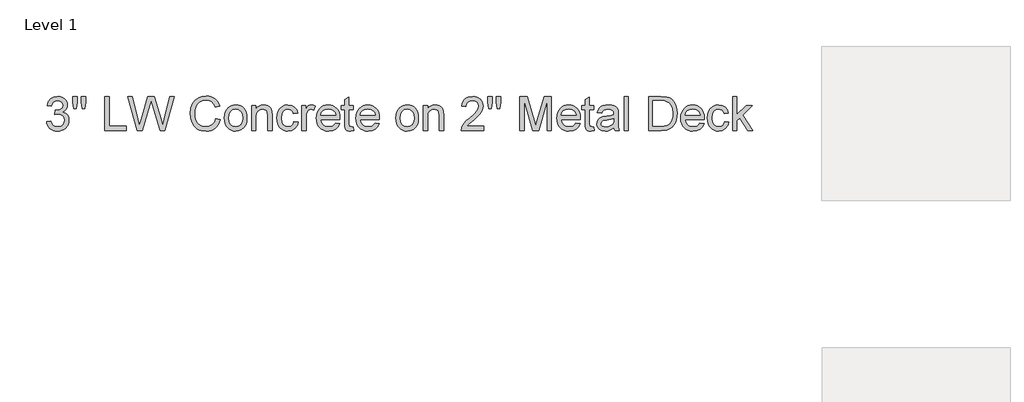
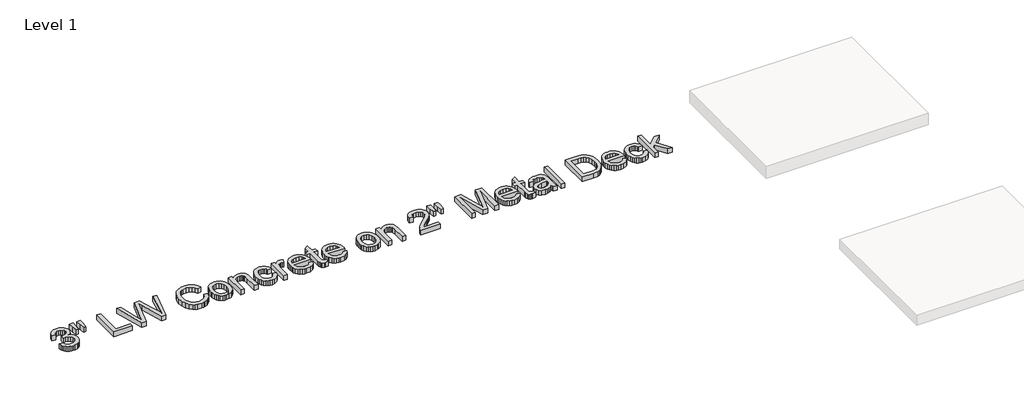
# One storey, part 17 of 42: 1 proxy.
"""IFC4 building model written with IfcOpenShell, lengths in millimetres."""

from ifc_helpers import new_model, si_unit, origin, origin_with_axes, place, context, project, spatial, polyline, outline, extrude, element, save

model = new_model("IFC4")

# Units and contexts
model_context = context("Model", 3, world=origin())
ifc_project = project(units=[si_unit("LENGTHUNIT", "METRE", prefix="MILLI")], contexts=[model_context])

# Site, building, storey
site = spatial("IfcSite", under=ifc_project)
building = spatial("IfcBuilding", under=site)
storey = spatial("IfcBuildingStorey", under=building, Name="Level 1", Elevation=0.0)

# Proxy
placement = place(None, origin())
element("IfcBuildingElementProxy", 1, Name="8\" Arial", ObjectType="8\" Arial", at=placement, inside=storey, context=model_context, shape_type="SweptSolid", body=[
    extrude(outline(polyline([(16880.3243613, -5919.794277), (16918.3952481, -5915.0354162), (16926.9184422, -5938.9598455), (16939.4011573, -5955.1139474), (16956.4568402, -5964.315651), (16978.6989378, -5967.3828855), (17004.7983153, -5963.1631143), (17024.9491167, -5950.5038009), (17037.8315017, -5931.6170719), (17042.12563, -5908.7150541), (17037.8686803, -5886.9748676), (17025.0978311, -5869.3429164), (17005.7649589, -5857.6595412), (16981.8219403, -5853.7650828), (16955.1277052, -5857.929086), (16959.3660657, -5819.8581993), (16965.4633561, -5820.3043425), (16988.2724274, -5817.5717154), (17008.6648897, -5809.373834), (17023.0530081, -5795.5062161), (17027.8490475, -5775.7643793), (17024.3728484, -5759.3221433), (17013.944251, -5745.9843204), (16998.03181, -5737.1451082), (16978.1040802, -5734.1987041), (16958.1391719, -5737.1729921), (16941.8177663, -5746.0958562), (16929.9020249, -5760.9672963), (16923.1541089, -5781.7873125), (16885.0832222, -5777.0284517), (16896.2925702, -5742.8427287), (16916.2388893, -5717.3196195), (16943.5279819, -5701.4257679), (16976.7656506, -5696.1278173), (17000.6993746, -5698.739614), (17022.6812221, -5706.575004), (17041.2147543, -5718.9368886), (17054.8035328, -5735.1281691), (17063.1408339, -5753.7825318), (17065.9199343, -5773.5336633), (17063.2802536, -5791.9370704), (17055.3612118, -5808.630262), (17042.2743444, -5822.8510766), (17024.1311875, -5833.837353), (17047.9626703, -5843.4666105), (17065.6225055, -5859.8623733), (17076.553014, -5882.1323549), (17080.1965168, -5909.3842689), (17078.3747654, -5928.6985518), (17072.9095111, -5946.4885121), (17063.800754, -5962.7541497), (17051.0484941, -5977.4954648), (17035.5124865, -5989.7272243), (17018.0524863, -5998.4641954), (16998.6684936, -6003.706378), (16977.3605082, -6005.4537722), (16958.1019933, -6003.9619809), (16940.5536939, -5999.4866069), (16924.7156101, -5992.0276502), (16910.587742, -5981.5851108), (16898.7417105, -5968.7724357), (16889.7491365, -5954.2030717), (16883.6100201, -5937.8770188), (16880.3243613, -5919.794277)])), origin_with_axes(), (0.0, 0.0, 1.0), 50.8),
    extrude(outline(polyline([(17198.7218947, -5805.5816168), (17189.6503162, -5746.765071), (17189.6503162, -5696.1278173), (17227.721203, -5696.1278173), (17227.721203, -5746.765071), (17218.7983389, -5805.5816168), (17198.7218947, -5805.5816168)])), origin_with_axes(), (0.0, 0.0, 1.0), 50.8),
    extrude(outline(polyline([(17122.8031928, -5805.5816168), (17113.5085427, -5746.765071), (17113.5085427, -5696.1278173), (17151.5794295, -5696.1278173), (17151.5794295, -5746.765071), (17143.251423, -5805.5816168), (17122.8031928, -5805.5816168)])), origin_with_axes(), (0.0, 0.0, 1.0), 50.8),
    extrude(outline(polyline([(17399.0401934, -6000.6949114), (17399.0401934, -5696.1278173), (17437.1110802, -5696.1278173), (17437.1110802, -5962.6240246), (17589.3946272, -5962.6240246), (17589.3946272, -6000.6949114), (17399.0401934, -6000.6949114)])), origin_with_axes(), (0.0, 0.0, 1.0), 50.8),
    extrude(outline(polyline([(17686.7282029, -6000.6949114), (17603.6712097, -5696.1278173), (17642.9318117, -5696.1278173), (17691.1152778, -5896.2974016), (17705.9867179, -5958.0882354), (17721.8991588, -5903.4356929), (17782.2772058, -5696.1278173), (17838.8630355, -5696.1278173), (17882.733784, -5846.4037199), (17901.5275664, -5902.1716205), (17915.3765951, -5958.0882354), (17929.801892, -5898.0819744), (17978.4315013, -5696.1278173), (18017.6921032, -5696.1278173), (17934.5607528, -6000.6949114), (17893.8873641, -6000.6949114), (17820.868593, -5765.7261572), (17810.6816565, -5732.9346317), (17799.2306476, -5772.4183052), (17732.6809529, -6000.6949114), (17686.7282029, -6000.6949114)])), origin_with_axes(), (0.0, 0.0, 1.0), 50.8),
    extrude(outline(polyline([(18388.8832491, -5892.4308272), (18426.9541359, -5902.2459777), (18419.420822, -5925.9217751), (18409.3872472, -5946.6093425), (18396.8534116, -5964.30868), (18381.8193151, -5979.0197874), (18364.6242124, -5990.5846558), (18345.6073583, -5998.845276), (18324.7687528, -6003.8016482), (18302.1083959, -6005.4537722), (18257.9495133, -6000.4532505), (18239.278885, -5994.2025983), (18222.8807986, -5985.4516852), (18196.0006705, -5960.9695769), (18176.4075481, -5927.5274259), (18164.4453335, -5888.211056), (18160.4579286, -5846.1062911), (18164.9658339, -5801.696453), (18178.4895497, -5763.3467268), (18200.3226828, -5732.2747115), (18229.7588396, -5709.6980065), (18264.6695454, -5695.951219), (18302.9263251, -5691.3689565), (18324.7013666, -5692.8514532), (18344.6685987, -5697.2989432), (18362.8280213, -5704.7114267), (18379.1796344, -5715.0889035), (18393.4538933, -5728.1571815), (18405.381253, -5743.6420686), (18422.195275, -5781.8616697), (18384.1243883, -5790.9332482), (18370.9259852, -5763.1701284), (18352.894364, -5744.1253904), (18329.8064532, -5733.11123), (18301.4391811, -5729.4398432), (18268.7406021, -5733.5109), (18241.8790633, -5745.7240702), (18221.4958957, -5764.7966922), (18208.23243, -5789.4461042), (18200.954719, -5817.3114652), (18198.5288153, -5846.0319339), (18201.4008622, -5881.2028899), (18210.0170028, -5911.614985), (18224.70255, -5936.1063879), (18245.7828164, -5953.5152675), (18271.05497, -5963.915981), (18298.3161787, -5967.3828855), (18330.0945873, -5962.6612032), (18356.5750454, -5948.4961565), (18376.5678378, -5925.0364597), (18388.8832491, -5892.4308272)])), origin_with_axes(), (0.0, 0.0, 1.0), 50.8),
    extrude(outline(polyline([(18465.0250226, -5888.8616815), (18467.0837876, -5859.8949045), (18473.2600826, -5834.9341217), (18483.5539076, -5813.9793331), (18497.9652626, -5797.0305387), (18512.4742113, -5786.197624), (18528.4888934, -5778.4598278), (18546.0093089, -5773.8171501), (18565.0354576, -5772.2695908), (18586.0390431, -5774.1540811), (18605.0303369, -5779.8075521), (18622.009339, -5789.2300036), (18636.9760493, -5802.4214357), (18649.1915431, -5818.9357053), (18657.9168959, -5838.326669), (18663.1521076, -5860.594327), (18664.8971781, -5885.7386791), (18661.8113543, -5924.1999412), (18652.5538828, -5953.4780889), (18637.3943085, -5975.4041685), (18616.6021763, -5991.8092259), (18591.906291, -6002.0426357), (18565.0354576, -6005.4537722), (18543.7251486, -6003.5762529), (18524.5572565, -5997.943695), (18507.5317812, -5988.5560984), (18492.6487227, -5975.4134632), (18480.5633539, -5958.7388609), (18471.9309477, -5938.7553632), (18466.7515039, -5915.4629701), (18465.0250226, -5888.8616815)]), holes=[polyline([(18503.0959094, -5888.7873243), (18507.5015735, -5923.2425922), (18520.718566, -5947.7897631), (18540.6091172, -5962.4846049), (18565.0354576, -5967.3828855), (18589.3502622, -5962.4567209), (18609.2036348, -5947.6782273), (18622.4206272, -5922.8057437), (18626.8262914, -5887.5976091), (18622.3927433, -5854.1461635), (18609.092099, -5829.9336), (18589.2108425, -5815.2387582), (18565.0354576, -5810.3404776), (18540.6091172, -5815.2201689), (18520.718566, -5829.8592428), (18507.5015735, -5854.3506458), (18503.0959094, -5888.7873243)])]), origin_with_axes(), (0.0, 0.0, 1.0), 50.8),
    extrude(outline(polyline([(18707.7269257, -6000.6949114), (18707.7269257, -5777.0284517), (18745.7978125, -5777.0284517), (18745.7978125, -5808.258476), (18759.0240996, -5792.5133387), (18774.9086566, -5781.2668121), (18793.4514835, -5774.5188962), (18814.6525803, -5772.2695908), (18833.4184789, -5774.0820476), (18850.6042869, -5779.5194179), (18864.9366373, -5787.9031923), (18875.1421631, -5798.5548613), (18886.5559934, -5826.5503474), (18888.5636378, -5863.3571617), (18888.5636378, -6000.6949114), (18850.4927511, -6000.6949114), (18850.4927511, -5868.4878085), (18846.1056762, -5834.8039966), (18840.0362697, -5824.7750692), (18830.6021999, -5816.9954471), (18818.5098601, -5812.00422), (18804.4656438, -5810.3404776), (18782.1677783, -5814.0769269), (18763.1602189, -5825.2862749), (18755.5641661, -5834.436858), (18750.1384141, -5846.9428096), (18745.7978125, -5882.0208191), (18745.7978125, -6000.6949114), (18707.7269257, -6000.6949114)])), origin_with_axes(), (0.0, 0.0, 1.0), 50.8),
    extrude(outline(polyline([(19083.6769325, -5919.794277), (19121.7478192, -5924.5531379), (19111.1333288, -5958.4135481), (19091.1870097, -5984.0017198), (19063.7863813, -6000.0907591), (19030.8089628, -6005.4537722), (19009.4568279, -6003.5832239), (18990.3121723, -5997.9715789), (18973.3749962, -5988.6188373), (18958.6452995, -5975.524999), (18946.7225871, -5958.9363722), (18938.206364, -5939.0992653), (18933.0966301, -5916.0136781), (18931.3933854, -5889.6796107), (18934.3026109, -5855.8006112), (18943.0302873, -5826.4388116), (18957.7158345, -5802.7281592), (18978.4986721, -5785.8026014), (19003.3618611, -5775.6528435), (19030.2884624, -5772.2695908), (19062.4572463, -5776.9169159), (19088.1755431, -5790.858891), (19106.6254235, -5813.3519442), (19116.9889584, -5843.6525035), (19078.9180716, -5848.4113644), (19072.0121466, -5831.8018247), (19061.2582365, -5819.8953779), (19047.2511988, -5812.7292027), (19030.5858912, -5810.3404776), (19005.9829524, -5815.0435705), (18986.4548926, -5829.1528494), (18973.7119273, -5853.4304754), (18969.4642722, -5888.6386099), (18973.6189808, -5924.3207716), (18986.0831066, -5948.6820495), (19005.2579697, -5962.7076765), (19029.5448904, -5967.3828855), (19049.2588432, -5964.4643654), (19065.4222397, -5955.708805), (19077.1799721, -5940.8931327), (19083.6769325, -5919.794277)])), origin_with_axes(), (0.0, 0.0, 1.0), 50.8),
    extrude(outline(polyline([(19155.0598451, -6000.6949114), (19155.0598451, -5777.0284517), (19188.3718711, -5777.0284517), (19188.3718711, -5810.117406), (19200.6779878, -5790.9332482), (19212.0174609, -5779.6309537), (19223.3941126, -5774.1099316), (19235.8117651, -5772.2695908), (19254.7728513, -5775.2067003), (19274.0313663, -5784.0180286), (19261.3162849, -5818.1479837), (19247.9319888, -5812.2923541), (19234.5476927, -5810.3404776), (19223.1803356, -5812.2179969), (19213.0212831, -5817.8505549), (19204.8141071, -5826.8105976), (19199.3023796, -5838.6705711), (19194.6736438, -5859.9367305), (19193.1307319, -5883.1361771), (19193.1307319, -6000.6949114), (19155.0598451, -6000.6949114)])), origin_with_axes(), (0.0, 0.0, 1.0), 50.8),
    extrude(outline(polyline([(19454.4219352, -5934.0708596), (19491.7492499, -5938.8297204), (19478.2998912, -5966.9553316), (19456.8385442, -5987.9798301), (19427.8485306, -6001.0852867), (19391.8131722, -6005.4537722), (19368.190819, -6003.5692819), (19347.1430839, -5997.915811), (19328.6699668, -5988.4933595), (19312.7714678, -5975.3019274), (19299.9866766, -5958.7086533), (19290.8546829, -5939.080676), (19285.3754867, -5916.4179954), (19283.549088, -5890.7206116), (19285.394076, -5864.1518543), (19290.9290401, -5840.7339834), (19300.1539803, -5820.4669989), (19313.0688966, -5803.3509007), (19328.9255697, -5789.7528277), (19346.9757802, -5780.0399183), (19367.219528, -5774.2121727), (19389.6568134, -5772.2695908), (19411.3714396, -5774.2075254), (19431.0087116, -5780.021329), (19448.5686293, -5789.7110017), (19464.0511927, -5803.2765435), (19476.6895931, -5820.3554631), (19485.717022, -5840.585269), (19491.1334793, -5863.9659613), (19492.9389651, -5890.49754), (19492.7158935, -5900.7588337), (19321.6199747, -5900.7588337), (19328.2098816, -5929.2562308), (19343.5181703, -5950.2063721), (19365.6115536, -5963.0887571), (19392.5567442, -5967.3828855), (19412.8190814, -5965.3938304), (19429.8840589, -5959.426665), (19443.7516769, -5949.1096034), (19454.4219352, -5934.0708596)]), holes=[polyline([(19321.6199747, -5862.6879469), (19454.8680784, -5862.6879469), (19449.7188422, -5842.5743241), (19439.6248522, -5828.1862058), (19417.4292278, -5814.8019096), (19389.508099, -5810.3404776), (19363.8455701, -5813.9003286), (19342.6258839, -5824.5798815), (19327.8752742, -5841.2265998), (19321.6199747, -5862.6879469)])]), origin_with_axes(), (0.0, 0.0, 1.0), 50.8),
    extrude(outline(polyline([(19611.9104862, -5968.9443867), (19616.6693471, -6001.8102694), (19588.1905392, -6005.4537722), (19569.9172572, -6003.8736817), (19556.2913001, -5999.1334102), (19546.6620426, -5991.8278152), (19540.3788592, -5982.5517544), (19536.9212493, -5966.6207242), (19535.7687127, -5939.3502208), (19535.7687127, -5815.0993384), (19507.2155477, -5815.0993384), (19507.2155477, -5777.0284517), (19535.7687127, -5777.0284517), (19535.7687127, -5722.673338), (19573.8395995, -5700.2918206), (19573.8395995, -5777.0284517), (19611.9104862, -5777.0284517), (19611.9104862, -5815.0993384), (19573.8395995, -5815.0993384), (19573.8395995, -5938.2348628), (19575.8472439, -5957.8651638), (19582.353499, -5964.8175621), (19595.3288305, -5967.3828855), (19611.9104862, -5968.9443867)])), origin_with_axes(), (0.0, 0.0, 1.0), 50.8),
    extrude(outline(polyline([(19806.5776377, -5934.0708596), (19843.9049524, -5938.8297204), (19830.4555938, -5966.9553316), (19808.9942467, -5987.9798301), (19780.0042331, -6001.0852867), (19743.9688747, -6005.4537722), (19720.3465215, -6003.5692819), (19699.2987864, -5997.915811), (19680.8256693, -5988.4933595), (19664.9271703, -5975.3019274), (19652.1423791, -5958.7086533), (19643.0103854, -5939.080676), (19637.5311892, -5916.4179954), (19635.7047905, -5890.7206116), (19637.5497785, -5864.1518543), (19643.0847426, -5840.7339834), (19652.3096829, -5820.4669989), (19665.2245991, -5803.3509007), (19681.0812722, -5789.7528277), (19699.1314827, -5780.0399183), (19719.3752306, -5774.2121727), (19741.8125159, -5772.2695908), (19763.5271421, -5774.2075254), (19783.1644141, -5780.021329), (19800.7243318, -5789.7110017), (19816.2068952, -5803.2765435), (19828.8452956, -5820.3554631), (19837.8727245, -5840.585269), (19843.2891819, -5863.9659613), (19845.0946676, -5890.49754), (19844.871596, -5900.7588337), (19673.7756772, -5900.7588337), (19680.3655841, -5929.2562308), (19695.6738728, -5950.2063721), (19717.7672561, -5963.0887571), (19744.7124467, -5967.3828855), (19764.9747839, -5965.3938304), (19782.0397614, -5959.426665), (19795.9073794, -5949.1096034), (19806.5776377, -5934.0708596)]), holes=[polyline([(19673.7756772, -5862.6879469), (19807.0237809, -5862.6879469), (19801.8745447, -5842.5743241), (19791.7805547, -5828.1862058), (19769.5849303, -5814.8019096), (19741.6638015, -5810.3404776), (19716.0012726, -5813.9003286), (19694.7815864, -5824.5798815), (19680.0309767, -5841.2265998), (19673.7756772, -5862.6879469)])]), origin_with_axes(), (0.0, 0.0, 1.0), 50.8),
    extrude(outline(polyline([(19992.6193538, -5888.8616815), (19994.6781188, -5859.8949045), (20000.8544138, -5834.9341217), (20011.1482388, -5813.9793331), (20025.5595937, -5797.0305387), (20040.0685425, -5786.197624), (20056.0832246, -5778.4598278), (20073.60364, -5773.8171501), (20092.6297888, -5772.2695908), (20113.6333743, -5774.1540811), (20132.6246681, -5779.8075521), (20149.6036701, -5789.2300036), (20164.5703805, -5802.4214357), (20176.7858743, -5818.9357053), (20185.5112271, -5838.326669), (20190.7464388, -5860.594327), (20192.4915093, -5885.7386791), (20189.4056855, -5924.1999412), (20180.148214, -5953.4780889), (20164.9886397, -5975.4041685), (20144.1965075, -5991.8092259), (20119.5006222, -6002.0426357), (20092.6297888, -6005.4537722), (20071.3194798, -6003.5762529), (20052.1515876, -5997.943695), (20035.1261123, -5988.5560984), (20020.2430539, -5975.4134632), (20008.1576851, -5958.7388609), (19999.5252788, -5938.7553632), (19994.3458351, -5915.4629701), (19992.6193538, -5888.8616815)]), holes=[polyline([(20030.6902406, -5888.7873243), (20035.0959047, -5923.2425922), (20048.3128972, -5947.7897631), (20068.2034483, -5962.4846049), (20092.6297888, -5967.3828855), (20116.9445934, -5962.4567209), (20136.797966, -5947.6782273), (20150.0149584, -5922.8057437), (20154.4206226, -5887.5976091), (20149.9870745, -5854.1461635), (20136.6864302, -5829.9336), (20116.8051737, -5815.2387582), (20092.6297888, -5810.3404776), (20068.2034483, -5815.2201689), (20048.3128972, -5829.8592428), (20035.0959047, -5854.3506458), (20030.6902406, -5888.7873243)])]), origin_with_axes(), (0.0, 0.0, 1.0), 50.8),
    extrude(outline(polyline([(20235.3212569, -6000.6949114), (20235.3212569, -5777.0284517), (20273.3921437, -5777.0284517), (20273.3921437, -5808.258476), (20286.6184308, -5792.5133387), (20302.5029877, -5781.2668121), (20321.0458147, -5774.5188962), (20342.2469115, -5772.2695908), (20361.0128101, -5774.0820476), (20378.1986181, -5779.5194179), (20392.5309685, -5787.9031923), (20402.7364943, -5798.5548613), (20414.1503246, -5826.5503474), (20416.157969, -5863.3571617), (20416.157969, -6000.6949114), (20378.0870823, -6000.6949114), (20378.0870823, -5868.4878085), (20373.7000074, -5834.8039966), (20367.6306009, -5824.7750692), (20358.1965311, -5816.9954471), (20346.1041913, -5812.00422), (20332.059975, -5810.3404776), (20309.7621095, -5814.0769269), (20290.75455, -5825.2862749), (20283.1584973, -5834.436858), (20277.7327453, -5846.9428096), (20273.3921437, -5882.0208191), (20273.3921437, -6000.6949114), (20235.3212569, -6000.6949114)])), origin_with_axes(), (0.0, 0.0, 1.0), 50.8),
    extrude(outline(polyline([(20773.0725324, -5962.6240246), (20773.0725324, -6000.6949114), (20573.2003769, -6000.6949114), (20577.2900229, -5974.4468195), (20586.6776195, -5953.9335268), (20600.4151124, -5934.033681), (20620.2870742, -5913.2043701), (20648.078078, -5889.9026823), (20689.1604314, -5853.4118861), (20713.8098434, -5826.4759902), (20726.1345494, -5804.6149731), (20730.2427848, -5783.3488137), (20726.3669157, -5764.2854864), (20714.7393084, -5748.438108), (20696.8656963, -5737.7585551), (20674.2518127, -5734.1987041), (20650.5039817, -5737.6749032), (20632.0541013, -5748.1035006), (20620.1476545, -5764.6665671), (20616.0301245, -5786.5461734), (20577.9592377, -5781.7873125), (20581.2332782, -5762.1337749), (20587.1888253, -5744.9619089), (20595.8258789, -5730.2717144), (20607.144439, -5718.0631915), (20620.8842555, -5708.4664653), (20636.7850781, -5701.6116609), (20675.0697419, -5696.1278173), (20695.4738225, -5697.6521399), (20713.6332451, -5702.2251078), (20729.5480097, -5709.8467209), (20743.2181163, -5720.5169792), (20754.1974217, -5733.4458374), (20762.0397827, -5747.8432504), (20766.7451993, -5763.7092181), (20768.3136715, -5781.0437405), (20766.6220452, -5799.25196), (20761.5471663, -5817.1441615), (20752.5406503, -5835.3430863), (20739.0541131, -5854.4714762), (20717.5555874, -5877.3084315), (20684.5131063, -5906.6330525), (20640.7167151, -5943.2539739), (20623.5402018, -5962.6240246), (20773.0725324, -5962.6240246)])), origin_with_axes(), (0.0, 0.0, 1.0), 50.8),
    extrude(outline(polyline([(20820.4380692, -5805.5816168), (20811.1434191, -5746.765071), (20811.1434191, -5696.1278173), (20849.2143059, -5696.1278173), (20849.2143059, -5746.765071), (20840.8862994, -5805.5816168), (20820.4380692, -5805.5816168)])), origin_with_axes(), (0.0, 0.0, 1.0), 50.8),
    extrude(outline(polyline([(20896.3567711, -5805.5816168), (20887.2851927, -5746.765071), (20887.2851927, -5696.1278173), (20925.3560794, -5696.1278173), (20925.3560794, -5746.765071), (20916.4332153, -5805.5816168), (20896.3567711, -5805.5816168)])), origin_with_axes(), (0.0, 0.0, 1.0), 50.8),
    extrude(outline(polyline([(21096.6750698, -6000.6949114), (21096.6750698, -5696.1278173), (21162.1837636, -5696.1278173), (21224.4950978, -5910.7970557), (21237.0614648, -5955.6344478), (21250.6688325, -5907.0791957), (21311.9391659, -5696.1278173), (21377.4478597, -5696.1278173), (21377.4478597, -6000.6949114), (21339.3769729, -6000.6949114), (21339.3769729, -5734.1987041), (21262.8634134, -6000.6949114), (21211.2595161, -6000.6949114), (21134.7459566, -5734.1987041), (21134.7459566, -6000.6949114), (21096.6750698, -6000.6949114)])), origin_with_axes(), (0.0, 0.0, 1.0), 50.8),
    extrude(outline(polyline([(21595.9093153, -5934.0708596), (21633.2366301, -5938.8297204), (21619.7872714, -5966.9553316), (21598.3259244, -5987.9798301), (21569.3359107, -6001.0852867), (21533.3005523, -6005.4537722), (21509.6781991, -6003.5692819), (21488.630464, -5997.915811), (21470.157347, -5988.4933595), (21454.258848, -5975.3019274), (21441.4740568, -5958.7086533), (21432.3420631, -5939.080676), (21426.8628669, -5916.4179954), (21425.0364681, -5890.7206116), (21426.8814562, -5864.1518543), (21432.4164203, -5840.7339834), (21441.6413605, -5820.4669989), (21454.5562768, -5803.3509007), (21470.4129498, -5789.7528277), (21488.4631603, -5780.0399183), (21508.7069082, -5774.2121727), (21531.1441935, -5772.2695908), (21552.8588198, -5774.2075254), (21572.4960918, -5780.021329), (21590.0560094, -5789.7110017), (21605.5385728, -5803.2765435), (21618.1769733, -5820.3554631), (21627.2044022, -5840.585269), (21632.6208595, -5863.9659613), (21634.4263453, -5890.49754), (21634.2032737, -5900.7588337), (21463.1073549, -5900.7588337), (21469.6972618, -5929.2562308), (21485.0055505, -5950.2063721), (21507.0989337, -5963.0887571), (21534.0441243, -5967.3828855), (21554.3064615, -5965.3938304), (21571.3714391, -5959.426665), (21585.239057, -5949.1096034), (21595.9093153, -5934.0708596)]), holes=[polyline([(21463.1073549, -5862.6879469), (21596.3554585, -5862.6879469), (21591.2062224, -5842.5743241), (21581.1122324, -5828.1862058), (21558.916608, -5814.8019096), (21530.9954791, -5810.3404776), (21505.3329502, -5813.9003286), (21484.1132641, -5824.5798815), (21469.3626544, -5841.2265998), (21463.1073549, -5862.6879469)])]), origin_with_axes(), (0.0, 0.0, 1.0), 50.8),
    extrude(outline(polyline([(21753.3978664, -5968.9443867), (21758.1567273, -6001.8102694), (21729.6779194, -6005.4537722), (21711.4046373, -6003.8736817), (21697.7786803, -5999.1334102), (21688.1494228, -5991.8278152), (21681.8662393, -5982.5517544), (21678.4086295, -5966.6207242), (21677.2560929, -5939.3502208), (21677.2560929, -5815.0993384), (21648.7029278, -5815.0993384), (21648.7029278, -5777.0284517), (21677.2560929, -5777.0284517), (21677.2560929, -5722.673338), (21715.3269797, -5700.2918206), (21715.3269797, -5777.0284517), (21753.3978664, -5777.0284517), (21753.3978664, -5815.0993384), (21715.3269797, -5815.0993384), (21715.3269797, -5938.2348628), (21717.3346241, -5957.8651638), (21723.8408791, -5964.8175621), (21736.8162107, -5967.3828855), (21753.3978664, -5968.9443867)])), origin_with_axes(), (0.0, 0.0, 1.0), 50.8),
    extrude(outline(polyline([(21934.2345785, -5972.1417463), (21916.0449483, -5987.7381692), (21897.3162284, -5997.943695), (21877.6208648, -6003.5762529), (21856.5313038, -6005.4537722), (21824.7157165, -6000.9365723), (21801.2467251, -5987.3849725), (21786.7749549, -5966.8066172), (21781.9510315, -5941.2091508), (21783.7727829, -5925.426835), (21789.2380372, -5911.0944845), (21797.6682848, -5898.8255464), (21808.3850163, -5889.2334675), (21835.0420728, -5876.7414578), (21867.9823127, -5871.0159534), (21906.9083073, -5864.9930201), (21934.0115069, -5857.929086), (21934.2345785, -5849.4523652), (21931.6134872, -5832.4617448), (21923.7502132, -5821.3453433), (21906.1647353, -5813.091694), (21881.6640376, -5810.3404776), (21858.9850914, -5812.1715237), (21843.1470077, -5817.6646619), (21832.3466243, -5827.8237144), (21824.7807791, -5843.6525035), (21786.7098923, -5838.8936427), (21793.3183885, -5818.0736265), (21803.1800123, -5801.7150423), (21817.2149339, -5789.2044433), (21836.3433238, -5779.9283825), (21859.7379581, -5774.1842888), (21886.5716129, -5772.2695908), (21912.308499, -5773.9612172), (21932.7102559, -5779.0360961), (21948.0929018, -5786.6670038), (21958.7724547, -5796.0267165), (21965.8549781, -5807.5985558), (21970.4465353, -5821.8658437), (21972.3054653, -5855.1778696), (21972.3054653, -5902.5434065), (21974.2387525, -5968.6841365), (21981.823187, -6000.6949114), (21943.7523002, -6000.6949114), (21937.6550097, -5987.4593297), (21934.2345785, -5972.1417463)]), holes=[polyline([(21934.2345785, -5895.9999728), (21872.8155307, -5907.6740533), (21840.0611838, -5913.845701), (21825.2269223, -5923.8839231), (21820.0219182, -5938.5322916), (21822.8567865, -5949.8531754), (21831.3613913, -5959.1292362), (21845.3498397, -5965.3194732), (21864.6362387, -5967.3828855), (21885.0844689, -5965.1056962), (21903.1532686, -5958.2741284), (21917.8016372, -5948.2080223), (21927.9885737, -5936.2272184), (21932.5057736, -5923.8839231), (21934.0115069, -5906.7817669), (21934.2345785, -5895.9999728)])]), origin_with_axes(), (0.0, 0.0, 1.0), 50.8),
    extrude(outline(polyline([(22024.6529346, -6000.6949114), (22024.6529346, -5696.1278173), (22062.7238213, -5696.1278173), (22062.7238213, -6000.6949114), (22024.6529346, -6000.6949114)])), origin_with_axes(), (0.0, 0.0, 1.0), 50.8),
    extrude(outline(polyline([(22243.5605334, -6000.6949114), (22243.5605334, -5696.1278173), (22348.627258, -5696.1278173), (22402.9823717, -5700.5148922), (22427.2599978, -5708.9730237), (22447.7454066, -5722.301552), (22468.8070837, -5745.5009986), (22483.8086489, -5774.3515925), (22492.7872809, -5808.2956546), (22495.7801582, -5846.7755059), (22493.7539245, -5879.4647903), (22487.6752233, -5908.2317323), (22478.4177518, -5932.7231353), (22466.8552071, -5952.5858025), (22453.5452682, -5968.2658772), (22439.0456141, -5980.2095026), (22422.3988958, -5989.0673041), (22402.6477643, -5995.4899073), (22353.6835477, -6000.6949114), (22243.5605334, -6000.6949114)]), holes=[polyline([(22281.6314202, -5962.6240246), (22348.999044, -5962.6240246), (22376.864405, -5961.2484164), (22398.0004393, -5957.1215918), (22413.9500588, -5950.4852116), (22426.2561756, -5941.5809368), (22439.4824626, -5925.1015222), (22449.4184436, -5903.7703003), (22455.6365645, -5877.4943245), (22457.7092714, -5846.1806483), (22453.6475094, -5804.6893303), (22441.4622231, -5774.0541637), (22423.4584859, -5753.0110759), (22401.9413709, -5740.2959945), (22380.0431753, -5735.7230267), (22347.9580432, -5734.1987041), (22281.6314202, -5734.1987041), (22281.6314202, -5962.6240246)])]), origin_with_axes(), (0.0, 0.0, 1.0), 50.8),
    extrude(outline(polyline([(22699.9650313, -5934.0708596), (22737.2923461, -5938.8297204), (22723.8429874, -5966.9553316), (22702.3816404, -5987.9798301), (22673.3916267, -6001.0852867), (22637.3562683, -6005.4537722), (22613.7339151, -6003.5692819), (22592.68618, -5997.915811), (22574.213063, -5988.4933595), (22558.314564, -5975.3019274), (22545.5297728, -5958.7086533), (22536.3977791, -5939.080676), (22530.9185829, -5916.4179954), (22529.0921841, -5890.7206116), (22530.9371722, -5864.1518543), (22536.4721363, -5840.7339834), (22545.6970765, -5820.4669989), (22558.6119928, -5803.3509007), (22574.4686658, -5789.7528277), (22592.5188763, -5780.0399183), (22612.7626242, -5774.2121727), (22635.1999095, -5772.2695908), (22656.9145358, -5774.2075254), (22676.5518078, -5780.021329), (22694.1117254, -5789.7110017), (22709.5942888, -5803.2765435), (22722.2326893, -5820.3554631), (22731.2601182, -5840.585269), (22736.6765755, -5863.9659613), (22738.4820613, -5890.49754), (22738.2589897, -5900.7588337), (22567.1630709, -5900.7588337), (22573.7529778, -5929.2562308), (22589.0612665, -5950.2063721), (22611.1546497, -5963.0887571), (22638.0998403, -5967.3828855), (22658.3621775, -5965.3938304), (22675.4271551, -5959.426665), (22689.294773, -5949.1096034), (22699.9650313, -5934.0708596)]), holes=[polyline([(22567.1630709, -5862.6879469), (22700.4111745, -5862.6879469), (22695.2619384, -5842.5743241), (22685.1679484, -5828.1862058), (22662.972324, -5814.8019096), (22635.0511951, -5810.3404776), (22609.3886662, -5813.9003286), (22588.1689801, -5824.5798815), (22573.4183704, -5841.2265998), (22567.1630709, -5862.6879469)])]), origin_with_axes(), (0.0, 0.0, 1.0), 50.8),
    extrude(outline(polyline([(22919.3187734, -5919.794277), (22957.3896602, -5924.5531379), (22946.7751698, -5958.4135481), (22926.8288507, -5984.0017198), (22899.4282222, -6000.0907591), (22866.4508037, -6005.4537722), (22845.0986688, -6003.5832239), (22825.9540133, -5997.9715789), (22809.0168371, -5988.6188373), (22794.2871404, -5975.524999), (22782.364428, -5958.9363722), (22773.8482049, -5939.0992653), (22768.738471, -5916.0136781), (22767.0352264, -5889.6796107), (22769.9444518, -5855.8006112), (22778.6721283, -5826.4388116), (22793.3576754, -5802.7281592), (22814.140513, -5785.8026014), (22839.003702, -5775.6528435), (22865.9303033, -5772.2695908), (22898.0990872, -5776.9169159), (22923.817384, -5790.858891), (22942.2672645, -5813.3519442), (22952.6307993, -5843.6525035), (22914.5599125, -5848.4113644), (22907.6539875, -5831.8018247), (22896.9000774, -5819.8953779), (22882.8930397, -5812.7292027), (22866.2277321, -5810.3404776), (22841.6247933, -5815.0435705), (22822.0967335, -5829.1528494), (22809.3537682, -5853.4304754), (22805.1061131, -5888.6386099), (22809.2608217, -5924.3207716), (22821.7249475, -5948.6820495), (22840.8998106, -5962.7076765), (22865.1867313, -5967.3828855), (22884.9006841, -5964.4643654), (22901.0640806, -5955.708805), (22912.821813, -5940.8931327), (22919.3187734, -5919.794277)])), origin_with_axes(), (0.0, 0.0, 1.0), 50.8),
    extrude(outline(polyline([(22990.7016861, -6000.6949114), (22990.7016861, -5696.1278173), (23028.7725728, -5696.1278173), (23028.7725728, -5859.7880161), (23114.1346392, -5777.0284517), (23166.7795373, -5777.0284517), (23080.3764701, -5860.8290169), (23171.5383982, -6000.6949114), (23127.0727922, -6000.6949114), (23053.0873775, -5887.3001803), (23028.7725728, -5910.8714129), (23028.7725728, -6000.6949114), (22990.7016861, -6000.6949114)])), origin_with_axes(), (0.0, 0.0, 1.0), 50.8),
])

save(model, "model.ifc")

# Revit data of these elements
# Element 1 (IfcBuildingElementProxy, "8\" Arial")
#   Phase Created = New Construction
